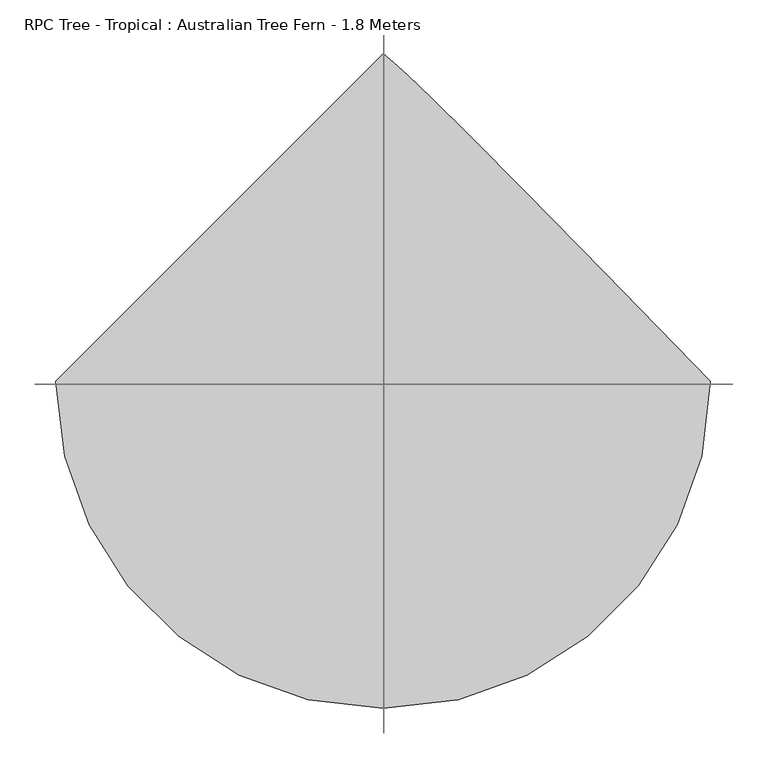
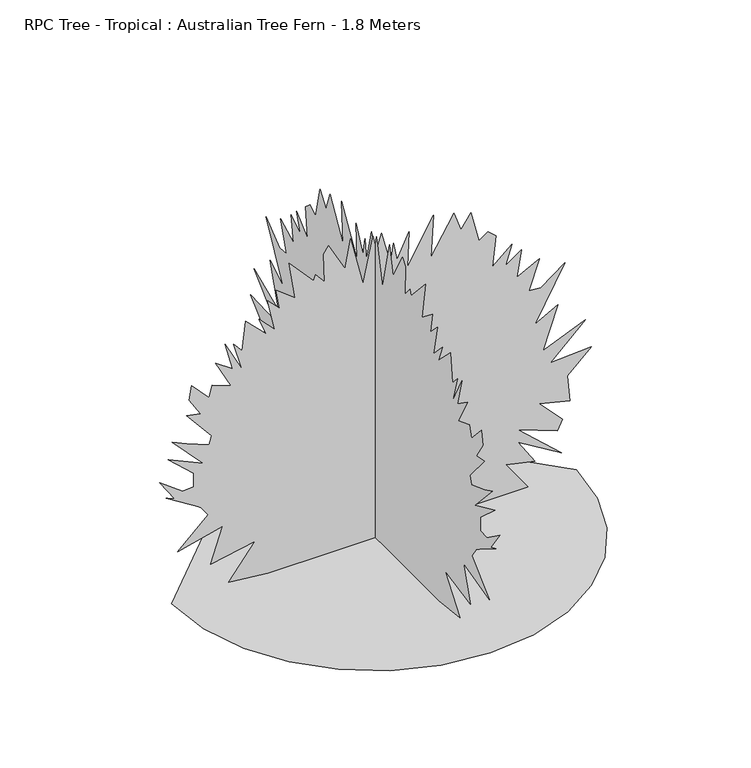
"""IFC4 building model written with IfcOpenShell, lengths in millimetres: geographic element geometry, RPC Tree - Tropical : Australian Tree Fern - 1.8 Meters."""

from ifc_helpers import new_model, si_unit, origin, place, context, project, spatial, triangles, source, transform, mapped, element, save


def rpc_tree_tropical_australian_tree_fern_1_8_meters_ded01fe0(model_context):
    return source(origin(), model_context, "Body", "Tessellation", [
        triangles([(-1121.4844528, 0.0, 0.0002091), (-1091.8312483, -257.014581, 0.0002091), (-1007.379063, -493.0422163, 0.0002091), (-874.8874409, -701.3197649, 0.0002091), (-701.1231199, -875.0840858, 0.0002091), (-492.845535, -1007.575708, 0.0002091), (-256.8179179, -1092.0278933, 0.0002091), (0.1967201, -1121.6810978, 0.0002091), (257.2112442, -1092.0278933, 0.0002091), (493.2388976, -1007.575708, 0.0002091), (701.5164099, -875.0840858, 0.0002091), (875.2807308, -701.3197649, 0.0002091), (1007.772353, -493.0422163, 0.0002091), (1092.2245382, -257.014581, 0.0002091), (1121.8777428, 9.81e-05, 0.0002091), (757.3559521, 373.9099531, 0.0002091), (487.118886, 649.203978, 0.0002091), (295.4501165, 842.3164639, 0.0002091), (166.6377574, 969.6837622, 0.0002091), (84.9673791, 1047.7439684, 0.0002091), (34.7249062, 1092.9297277, 0.0002091), (0.196524, 1121.6810978, 0.0002091), (-584.7020648, -9.9524755, 0.0280128), (-811.2515722, -9.9524573, 23.5990138), (-664.9373926, -9.9524755, 212.3913055), (-910.368124, -9.9524755, 165.1928965), (-844.2910526, -9.9524755, 363.42491), (-1094.439374, -9.9524755, 302.0672271), (-924.5263441, -9.9524948, 457.820202), (-967.0045652, -9.9524948, 519.177903), (-1155.7970387, -9.9524948, 637.1720089), (-1108.5994108, -9.9524948, 618.292638), (-1193.5540363, -9.9524948, 741.0079674), (-1066.121117, -9.9524948, 646.6127117), (-1004.7634523, -9.9524948, 651.3321184), (-1004.7634523, -9.9524948, 731.5673372), (-1146.3564085, -9.952513, 859.002146), (-952.8445284, -9.952513, 769.3262243), (-1122.7575583, -9.952513, 953.399291), (-1042.5223394, -9.952513, 915.6404039), (-919.8069374, -9.952513, 868.4427761), (-905.6469006, -9.952513, 915.6404039), (-1042.5223394, -9.952513, 1080.8322104), (-967.0045652, -9.952513, 1066.6740629), (-1028.3623026, -9.9525323, 1165.7887253), (-1014.2022657, -9.9525323, 1246.0258335), (-919.8069374, -9.9525323, 1142.1899477), (-900.9274939, -9.9525323, 1208.2670191), (-797.0915354, -9.9525323, 1170.508132), (-882.0480503, -9.9525323, 1330.9824211), (-787.652722, -9.9525323, 1264.9053497), (-830.1310158, -9.9525504, 1425.3776768), (-735.7356874, -9.9525323, 1246.0258335), (-782.9333879, -9.9525504, 1406.4983059), (-735.7356874, -9.9525323, 1354.5812714), (-716.8562439, -9.9525504, 1519.7729324), (-603.5815084, -9.9525504, 1406.4983059), (-641.3385424, -9.9525504, 1505.614785), (-556.3819911, -9.9525504, 1415.9388634), (-594.1408419, -9.9525504, 1595.2907066), (-528.0637705, -9.9525504, 1529.2136353), (-546.943214, -9.9525504, 1642.4884071), (-443.1072556, -9.9525504, 1562.2512989), (-476.146736, -9.9525697, 1774.6425499), (-339.2712971, -9.9525504, 1623.6088909), (-329.83252, -9.9525504, 1656.648444), (-279.7754919, -9.9525504, 1596.614463), (-284.4967516, -9.9525697, 1761.8062695), (-256.1691566, -9.9525697, 1800.0058273), (-164.5496218, -9.9525697, 1634.348933), (-134.8663864, -9.9525323, 1797.6189091), (-66.8546674, -9.9525323, 1511.5436382), (-8.8864392, -9.9525697, 1769.9232159), (9.9927528, -9.9525504, 1680.2472942), (38.3116059, -9.9525697, 1769.9232159), (85.5096334, -9.9525504, 1576.4113358), (104.3886955, -9.9525504, 1689.6861076), (123.2679392, -9.9525504, 1585.8501492), (189.3454011, -9.9525697, 1727.4448494), (179.9054977, -9.9525504, 1524.4943012), (326.2189688, -9.9525697, 1774.6425499), (312.0589319, -9.9525504, 1533.9331146), (439.4937043, -9.9525697, 1746.3243656), (477.2525914, -9.9525504, 1637.7690731), (533.8908857, -9.9525697, 1718.0042919), (576.3691432, -9.9525504, 1538.6524487), (628.2861414, -9.9525504, 1571.6918564), (670.7644352, -9.9525504, 1533.9331146), (651.8849916, -9.9525323, 1359.3006054), (760.4403568, -9.9525504, 1453.6958611), (722.6814697, -9.9525323, 1340.4212345), (812.3573914, -9.9525504, 1401.7788265), (788.7585411, -9.9525323, 1250.7453129), (911.4739431, -9.9525323, 1316.8223843), (854.8356125, -9.9525323, 1146.9092817), (920.9127565, -9.9525323, 1142.1899477), (1053.0668993, -9.9525323, 1241.3064995), (887.8750929, -9.952513, 939.2392542), (1015.3099016, -9.952513, 1010.0357323), (930.3533867, -9.952513, 769.3262243), (1166.3416712, -9.952513, 868.4427761), (972.8316078, -9.9524948, 684.3697094), (1199.3811516, -9.9524948, 698.5297462), (1067.2269361, -9.9524948, 575.8143442), (1081.386973, -9.9524755, 424.7807216), (911.4739431, -9.9524948, 467.2590154), (1038.9087519, -9.9524755, 330.3854296), (1010.5886055, -9.9524755, 273.7490065), (793.4779478, -9.9524755, 353.9842435), (1034.1874557, -9.9524755, 136.8741308), (793.4779478, -9.9524755, 283.1877836), (887.8750929, -9.9524755, 136.8741308), (727.4008764, -9.9524755, 174.6324366), (850.2137289, -9.9524755, 0.0285496), (14.7125365, -9.9524573, 9.11e-05), (2.9132547, -597.5662868, 0.0279397), (2.913236, -824.1176474, 23.5990138), (2.9132547, -677.8033951, 212.3913055), (2.9132547, -923.2323097, 165.1928965), (2.9132547, -857.1552383, 363.42491), (2.9132547, -1107.3054491, 302.0672271), (2.9132547, -937.3923466, 457.820202), (2.9132547, -979.8706404, 519.177903), (2.9132735, -1168.6612244, 637.1720089), (2.9132735, -1121.4635965, 618.292638), (2.9132735, -1206.4201115, 741.0079674), (2.9132735, -1078.9853027, 646.6127117), (2.9132735, -1017.6295275, 651.3321184), (2.9132735, -1017.6295275, 731.5673372), (2.9132735, -1159.2224836, 859.002146), (2.9132735, -965.7106035, 769.3262243), (2.9132735, -1135.6236334, 953.399291), (2.9132735, -1055.3865252, 915.6404039), (2.9132735, -932.6730125, 868.4427761), (2.9132735, -918.5129757, 915.6404039), (2.9132735, -1055.3865252, 1080.8322104), (2.9132735, -979.8706404, 1066.6740629), (2.9132735, -1041.2283051, 1165.7887253), (2.9132922, -1027.0682682, 1246.0258335), (2.9132735, -932.6730125, 1142.1899477), (2.9132735, -913.793569, 1208.2670191), (2.9132735, -809.9576105, 1170.5100214), (2.9132922, -894.9141254, 1330.9824211), (2.9132735, -800.5187971, 1264.9053497), (2.9132922, -842.9970909, 1425.3776768), (2.9132735, -748.5998732, 1246.0258335), (2.9132922, -795.7975737, 1406.4983059), (2.9132735, -748.5998732, 1354.5812714), (2.9132922, -729.722319, 1519.7729324), (2.9132735, -616.4457304, 1406.4983059), (2.9132922, -654.2046175, 1505.614785), (2.9132735, -569.2480662, 1415.9388634), (2.9132922, -607.0069533, 1595.2907066), (2.9132922, -540.9298456, 1529.2136353), (2.9132922, -559.8092892, 1642.4884071), (2.9132922, -455.9733307, 1562.2512989), (2.9132922, -489.010958, 1774.6425499), (2.9132922, -352.1373722, 1623.6088909), (2.9132922, -342.6985951, 1656.648444), (2.9132922, -292.641567, 1596.614463), (2.9132922, -297.3609555, 1761.8062695), (2.9132922, -269.0352317, 1800.0058273), (2.9132922, -177.4153154, 1634.348933), (2.9132547, -147.7320982, 1797.6189091), (2.9132547, -79.72057, 1511.5455276), (2.9132922, -21.7521334, 1769.9232159), (2.9132735, -2.872978, 1680.2472942), (2.9132922, 25.4458941, 1769.9232159), (2.9132735, 72.6439216, 1576.4113358), (2.9132735, 91.5229837, 1689.6861076), (2.9132735, 110.4020457, 1585.8518932), (2.9132735, 176.4793078, 1727.4448494), (2.9132735, 167.0397859, 1524.4943012), (2.9132735, 313.3528936, 1774.6425499), (2.9132735, 299.1947099, 1533.9331146), (2.9132735, 426.6276292, 1746.3243656), (2.9132735, 464.3864799, 1637.7690731), (2.9132735, 521.0248106, 1718.0061813), (2.9132735, 563.5030681, 1538.6524487), (2.9132735, 615.4200663, 1571.6918564), (2.9132735, 657.8983601, 1533.9331146), (2.9132547, 639.0189165, 1359.3006054), (2.9132547, 747.5742817, 1453.6958611), (2.9132547, 709.8153946, 1340.4212345), (2.9132547, 799.4913162, 1401.7788265), (2.9132547, 775.892466, 1250.7453129), (2.9132547, 898.607868, 1316.8223843), (2.9132547, 841.96961, 1146.9092817), (2.9132547, 908.0466814, 1142.1899477), (2.9132547, 1040.2008242, 1241.3064995), (2.9132547, 875.0090904, 939.2392542), (2.9132547, 1002.4438265, 1010.0357323), (2.913236, 917.4873116, 769.3262243), (2.913236, 1153.4774855, 868.4427761), (2.913236, 959.9656054, 684.3697094), (2.913236, 1186.5150764, 698.5297462), (2.913236, 1054.360861, 575.8143442), (2.913236, 1068.5208979, 424.7807216), (2.913236, 898.607868, 467.2590154), (2.9132173, 1026.0426767, 330.3854296), (2.9132173, 997.7244198, 273.7490065), (2.913236, 780.6137621, 353.9842435), (2.9132173, 1021.32327, 136.8739401), (2.913236, 780.6137621, 283.1877836), (2.9132173, 875.0090904, 136.8739401), (2.9132173, 714.5366907, 174.6324366), (2.913236, 837.3476538, 0.0284335), (2.913236, 1.8467684, 0.0)], [[21, 22, 1], [20, 21, 1], [19, 20, 1], [18, 19, 1], [17, 18, 1], [17, 1, 2], [17, 2, 3], [17, 3, 4], [16, 17, 4], [16, 4, 5], [16, 5, 6], [16, 6, 7], [16, 7, 8], [16, 8, 9], [16, 9, 10], [16, 10, 11], [16, 11, 12], [15, 16, 12], [14, 15, 12], [13, 14, 12], [30, 31, 32], [109, 110, 111], [51, 52, 53], [36, 37, 38], [32, 33, 34], [76, 77, 78], [100, 101, 102], [38, 39, 40], [78, 79, 80], [57, 58, 59], [70, 71, 72], [96, 97, 98], [72, 73, 74], [53, 54, 55], [80, 81, 82], [49, 50, 51], [27, 28, 29], [89, 90, 91], [74, 75, 76], [59, 60, 61], [63, 64, 65], [38, 40, 41], [102, 103, 104], [42, 43, 44], [98, 99, 100], [61, 62, 63], [93, 94, 95], [111, 112, 113], [91, 92, 93], [84, 85, 86], [82, 83, 84], [55, 56, 57], [45, 46, 47], [44, 45, 47], [113, 114, 115], [65, 66, 67], [23, 24, 25], [72, 74, 76], [25, 26, 27], [68, 69, 70], [67, 68, 70], [30, 32, 34], [30, 34, 35], [104, 105, 106], [49, 51, 53], [102, 104, 106], [95, 96, 98], [47, 48, 49], [107, 108, 109], [106, 107, 109], [82, 84, 86], [86, 87, 88], [86, 88, 89], [67, 70, 72], [115, 23, 25], [53, 55, 57], [82, 86, 89], [76, 78, 80], [63, 65, 67], [59, 61, 63], [42, 44, 47], [42, 47, 49], [35, 36, 38], [72, 76, 80], [111, 113, 115], [109, 111, 115], [100, 102, 106], [100, 106, 109], [100, 109, 115], [98, 100, 115], [98, 115, 25], [95, 98, 25], [93, 95, 25], [91, 93, 25], [89, 91, 25], [82, 89, 25], [80, 82, 25], [72, 80, 25], [72, 25, 27], [72, 27, 29], [67, 72, 29], [63, 67, 29], [59, 63, 29], [59, 29, 30], [59, 30, 35], [59, 35, 38], [59, 38, 41], [59, 41, 42], [59, 42, 49], [59, 49, 53], [59, 53, 57], [123, 124, 125], [202, 203, 204], [144, 145, 146], [129, 130, 131], [125, 126, 127], [169, 170, 171], [193, 194, 195], [131, 132, 133], [171, 172, 173], [150, 151, 152], [163, 164, 165], [189, 190, 191], [165, 166, 167], [146, 147, 148], [173, 174, 175], [142, 143, 144], [120, 121, 122], [182, 183, 184], [167, 168, 169], [152, 153, 154], [156, 157, 158], [131, 133, 134], [195, 196, 197], [135, 136, 137], [191, 192, 193], [154, 155, 156], [186, 187, 188], [204, 205, 206], [184, 185, 186], [177, 178, 179], [175, 176, 177], [148, 149, 150], [138, 139, 140], [137, 138, 140], [206, 207, 208], [158, 159, 160], [116, 117, 118], [165, 167, 169], [118, 119, 120], [161, 162, 163], [160, 161, 163], [123, 125, 127], [123, 127, 128], [197, 198, 199], [142, 144, 146], [195, 197, 199], [188, 189, 191], [140, 141, 142], [200, 201, 202], [199, 200, 202], [175, 177, 179], [179, 180, 181], [179, 181, 182], [160, 163, 165], [208, 116, 118], [146, 148, 150], [175, 179, 182], [169, 171, 173], [156, 158, 160], [152, 154, 156], [135, 137, 140], [135, 140, 142], [128, 129, 131], [165, 169, 173], [204, 206, 208], [202, 204, 208], [193, 195, 199], [193, 199, 202], [193, 202, 208], [191, 193, 208], [191, 208, 118], [188, 191, 118], [186, 188, 118], [184, 186, 118], [182, 184, 118], [175, 182, 118], [173, 175, 118], [165, 173, 118], [165, 118, 120], [165, 120, 122], [160, 165, 122], [156, 160, 122], [152, 156, 122], [152, 122, 123], [152, 123, 128], [152, 128, 131], [152, 131, 134], [152, 134, 135], [152, 135, 142], [152, 142, 146], [152, 146, 150]], closed=False),
    ])


if __name__ == "__main__":
    model = new_model("IFC4")
    model_context = context("Model", 3, world=origin())
    ifc_project = project(units=[si_unit("LENGTHUNIT", "METRE", prefix="MILLI")], contexts=[model_context])
    site = spatial("IfcSite", under=ifc_project)
    building = spatial("IfcBuilding", under=site)
    placement = place(None, origin())
    rpc_tree_tropical_australian_tree_fern_1_8_meters_shape = rpc_tree_tropical_australian_tree_fern_1_8_meters_ded01fe0(model_context)
    element("IfcGeographicElement", 1, ObjectType="RPC Tree - Tropical : Australian Tree Fern - 1.8 Meters", at=placement, inside=building, context=model_context, shape_type="MappedRepresentation", body=[
        mapped(rpc_tree_tropical_australian_tree_fern_1_8_meters_shape, transform((0.0, 0.0, 0.0), x_axis=(1.0, 0.0, 0.0), y_axis=(0.0, 1.0, 0.0), z_axis=(0.0, 0.0, 1.0))),
    ])
    save(model, "model.ifc")

# Revit data of these elements
# Type "RPC Tree - Tropical : Australian Tree Fern - 1.8 Meters"
#   built-in parameter 1005195 = "RPC-16-G2F6-877X-GLVN-N000-ST1L-LVER-AU"
#   Type Comments = "Australian Tree Fern"
#   Height = 1800 mm
#   Plan Symbol = element 242927
#   Description = (empty or 0)
